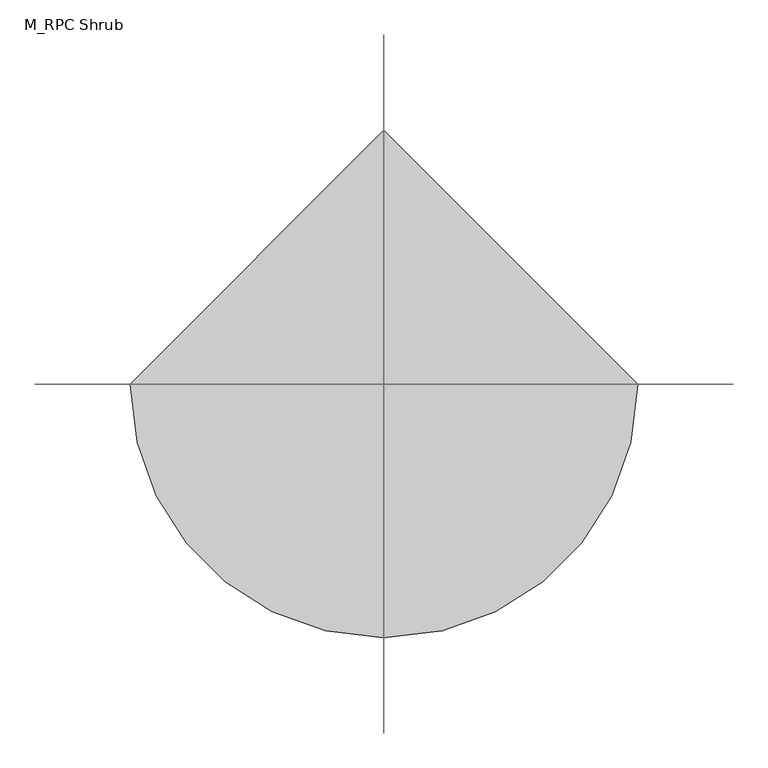
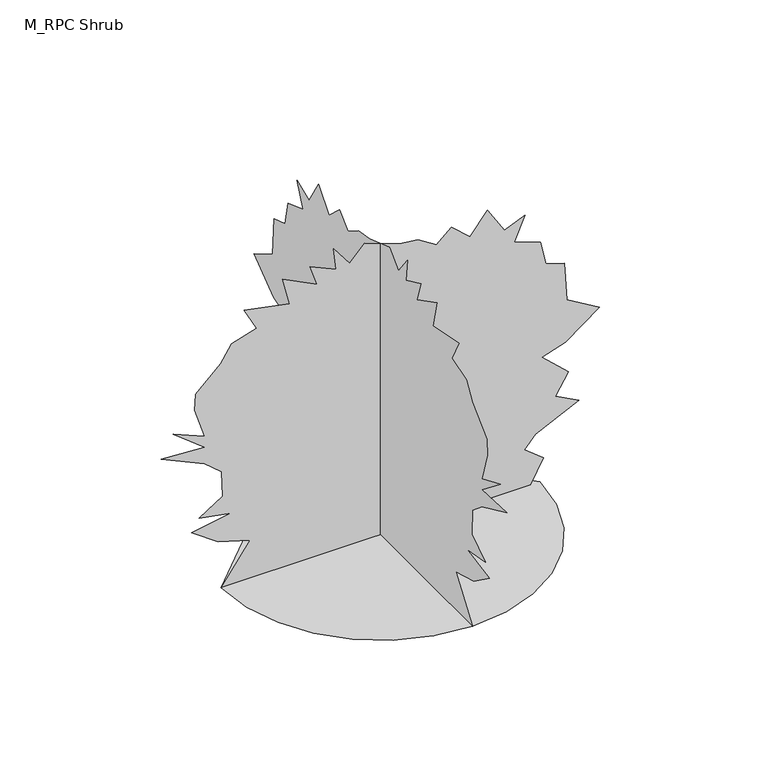
"""IFC4 building model written with IfcOpenShell, lengths in millimetres: geographic element geometry, M_RPC Shrub : Oleander - 1.62 Meters."""

import ifcopenshell
import ifcopenshell.guid

model = None  # the IFC model being written
_history = None  # IfcOwnerHistory: only IFC2X3 demands one
_inside = {}  # id of a spatial element -> (the spatial element, [elements in it])
_under = {}  # id of a project, library or spatial element -> (it, [spatial elements below it])
_declared = {}  # id of a project -> (the project, [libraries it declares])
_typed = {}  # id of a type object -> (the type object, [elements of that type])
_made_of = {}  # id of a material, layer set ... -> (it, [elements and type objects made of it])


def new_model(schema):
    """Start an empty IFC model of exactly this schema.

    Asked for "IFC4X3", IfcOpenShell would pick the latest addendum, in which some entities
    have other attributes; the version numbers below select the first issue.
    IFC2X3 requires an IfcOwnerHistory on every rooted entity: one is made here for all.
    """
    global model, _history
    if schema == "IFC4X3":
        model = ifcopenshell.file(schema_version=(4, 3, 0, 0))
    else:
        model = ifcopenshell.file(schema=schema)
    _inside.clear()
    _under.clear()
    _declared.clear()
    _typed.clear()
    _made_of.clear()
    _history = None
    if model.schema == "IFC2X3":
        org = make("IfcOrganization", Name="unknown")
        user = make(
            "IfcPersonAndOrganization",
            ThePerson=make("IfcPerson", FamilyName="unknown"),
            TheOrganization=org,
        )
        app = make(
            "IfcApplication",
            ApplicationDeveloper=org,
            Version="unknown",
            ApplicationFullName="unknown",
            ApplicationIdentifier="unknown",
        )
        _history = make(
            "IfcOwnerHistory",
            OwningUser=user,
            OwningApplication=app,
            ChangeAction="ADDED",
            CreationDate=0,
        )
    return model


def make(cls, **values):
    """One entity of the class cls with the attributes given. An attribute that is None is left unset."""
    return model.create_entity(
        cls, **{name: value for name, value in values.items() if value is not None}
    )


def rooted(cls, **values):
    """An entity with a GlobalId (a new one), such as an element, a storey or a relation."""
    return make(cls, GlobalId=ifcopenshell.guid.new(), OwnerHistory=_history, **values)


def si_unit(unit_type, name, prefix=None):
    """IfcSIUnit, for example si_unit("LENGTHUNIT", "METRE", prefix="MILLI")."""
    return make("IfcSIUnit", UnitType=unit_type, Prefix=prefix, Name=name)


def assignment(units):
    """IfcUnitAssignment: the units of a project."""
    return None if units is None else make("IfcUnitAssignment", Units=units)


def point(xyz):
    """IfcCartesianPoint."""
    return None if xyz is None else make("IfcCartesianPoint", Coordinates=xyz)


def direction(xyz):
    """IfcDirection."""
    return None if xyz is None else make("IfcDirection", DirectionRatios=xyz)


def frame(location, z_axis=None, x_axis=None):
    """IfcAxis2Placement3D, a coordinate frame: its origin and axes. An axis left out is left unset."""
    return make(
        "IfcAxis2Placement3D",
        Location=point(location),
        Axis=direction(z_axis),
        RefDirection=direction(x_axis),
    )


def origin():
    """The frame at (0, 0, 0) with its axes left unset."""
    return frame((0.0, 0.0, 0.0))


def place(relative_to, where):
    """IfcLocalPlacement: puts the frame where relative to a parent placement (None: the world)."""
    return make(
        "IfcLocalPlacement", PlacementRelTo=relative_to, RelativePlacement=where
    )


def context(
    kind, dimensions, precision=None, world=None, true_north=None, identifier=None
):
    """IfcGeometricRepresentationContext, for example the 3D "Model" context."""
    return make(
        "IfcGeometricRepresentationContext",
        ContextIdentifier=identifier,
        ContextType=kind,
        CoordinateSpaceDimension=dimensions,
        Precision=precision,
        WorldCoordinateSystem=world,
        TrueNorth=true_north,
    )


def project(units=None, contexts=None):
    """IfcProject with its units and contexts."""
    return rooted(
        "IfcProject",
        Name="project",
        RepresentationContexts=contexts,
        UnitsInContext=assignment(units),
    )


def spatial(cls, under=None, at=None, **own):
    """A site, building, storey or space (cls), placed at a placement, below another one or the project."""
    s = rooted(cls, ObjectPlacement=at, **own)
    if under is not None:
        _under.setdefault(under.id(), (under, []))[1].append(s)
    return s


def point_list(points):
    """IfcCartesianPointList2D or 3D."""
    cls = (
        "IfcCartesianPointList2D" if len(points[0]) == 2 else "IfcCartesianPointList3D"
    )
    return make(cls, CoordList=points)


def triangles(points, corners, closed=None, point_numbers=None):
    """IfcTriangulatedFaceSet: each triangle names its three corners, points numbered from 1."""
    return make(
        "IfcTriangulatedFaceSet",
        Coordinates=point_list(points),
        Closed=closed,
        CoordIndex=corners,
        PnIndex=point_numbers,
    )


def shape(context_of_items, identifier, shape_type, items):
    """IfcShapeRepresentation: the items that make up one representation, for example the "Body"."""
    return make(
        "IfcShapeRepresentation",
        ContextOfItems=context_of_items,
        RepresentationIdentifier=identifier,
        RepresentationType=shape_type,
        Items=items,
    )


def source(mapping_origin, context_of_items, identifier, shape_type, items):
    """IfcRepresentationMap: a shape defined once, which mapped items show again and again."""
    return make(
        "IfcRepresentationMap",
        MappingOrigin=mapping_origin,
        MappedRepresentation=shape(context_of_items, identifier, shape_type, items),
    )


def transform(
    local_origin,
    x_axis=None,
    y_axis=None,
    z_axis=None,
    scale=None,
    scale2=None,
    scale3=None,
    uniform=True,
):
    """IfcCartesianTransformationOperator3D, or its non-uniform kind. x_axis, y_axis, z_axis: its Axis1, 2, 3."""
    if uniform:
        return make(
            "IfcCartesianTransformationOperator3D",
            Axis1=direction(x_axis),
            Axis2=direction(y_axis),
            LocalOrigin=point(local_origin),
            Scale=scale,
            Axis3=direction(z_axis),
        )
    return make(
        "IfcCartesianTransformationOperator3DnonUniform",
        Axis1=direction(x_axis),
        Axis2=direction(y_axis),
        LocalOrigin=point(local_origin),
        Scale=scale,
        Axis3=direction(z_axis),
        Scale2=scale2,
        Scale3=scale3,
    )


def mapped(mapping_source, mapping_target):
    """IfcMappedItem: shows the shape of a source again, moved by a transform."""
    return make(
        "IfcMappedItem", MappingSource=mapping_source, MappingTarget=mapping_target
    )


def made_of(thing, what):
    """Note that an element or type object is made of a material, layer set ...; save() writes the relation."""
    if what is not None:
        _made_of.setdefault(what.id(), (what, []))[1].append(thing)
    return thing


def element(
    cls,
    number,
    at=None,
    inside=None,
    cuts=None,
    type_object=None,
    material=None,
    context=None,
    identifier="Body",
    shape_type=None,
    held_by="IfcProductDefinitionShape",
    body=None,
    shapes=None,
    **own,
):
    """One element of the class cls, such as IfcWall. Its Tag is "e" and its number.

    at: its placement. inside: the storey or other place that contains it. cuts: it is an
    opening in that element (IfcRelVoidsElement). A single representation is given by context,
    identifier, shape_type and body (its items); several are given by shapes. held_by: the class
    of the entity that holds the representations. save() writes the other relations.
    """
    e = rooted(cls, Tag="e%d" % number, ObjectPlacement=at, **own)
    if body is not None:
        shapes = [shape(context, identifier, shape_type, body)]
    if shapes is not None:
        e.Representation = make(held_by, Representations=shapes)
    if inside is not None:
        _inside.setdefault(inside.id(), (inside, []))[1].append(e)
    if cuts is not None:
        rooted(
            "IfcRelVoidsElement", RelatingBuildingElement=cuts, RelatedOpeningElement=e
        )
    if type_object is not None:
        _typed.setdefault(type_object.id(), (type_object, []))[1].append(e)
    return made_of(e, material)


def aggregate(whole, parts):
    """IfcRelAggregates: a whole, such as a stair, and the parts it consists of."""
    return rooted("IfcRelAggregates", RelatingObject=whole, RelatedObjects=parts)


def save(model, path):
    """Write the relations noted so far, then the file.

    IfcRelAggregates (storeys below a building ...), IfcRelContainedInSpatialStructure (elements
    in a storey), IfcRelDefinesByType, IfcRelAssociatesMaterial and IfcRelDeclares: one each for
    every whole, place, type object, material and project.
    """
    for whole, parts in _under.values():
        aggregate(whole, parts)
    for where, things in _inside.values():
        rooted(
            "IfcRelContainedInSpatialStructure",
            RelatedElements=things,
            RelatingStructure=where,
        )
    for kind, things in _typed.values():
        rooted("IfcRelDefinesByType", RelatedObjects=things, RelatingType=kind)
    for what, things in _made_of.values():
        rooted("IfcRelAssociatesMaterial", RelatedObjects=things, RelatingMaterial=what)
    for by, libraries in _declared.values():
        rooted("IfcRelDeclares", RelatingContext=by, RelatedDefinitions=libraries)
    model.write(path)


def m_rpc_shrub_9f7608c0(model_context):
    return source(origin(), model_context, "Body", "Tessellation", [
        triangles([(-809.7417807, 0.0, 3.61e-05), (-788.3350204, -185.5390928, 3.61e-05), (-727.3673029, -355.9266395, 3.61e-05), (-631.7240129, -506.2829052, 3.61e-05), (-506.2829052, -631.7240129, 3.61e-05), (-355.9266395, -727.3673029, 3.61e-05), (-185.5390928, -788.3350204, 3.61e-05), (3.54e-05, -809.7417807, 3.61e-05), (185.5390928, -788.3350204, 3.61e-05), (355.9266395, -727.3673029, 3.61e-05), (506.2829052, -631.7240129, 3.61e-05), (631.7240129, -506.2829052, 3.61e-05), (727.3673029, -355.9266395, 3.61e-05), (788.3350204, -185.5390928, 3.61e-05), (809.7417807, 7.08e-05, 3.61e-05), (-0.0001062, 809.7417807, 3.61e-05), (-0.00426, -808.5039928, 0.0001204), (-0.0042561, -663.4380655, 203.8035848), (-0.0042523, -825.0482592, 250.5848863), (-0.0042473, -961.1383535, 348.4012267), (-0.0042493, -761.2531706, 382.4237866), (-0.004246, -922.8633642, 412.1938082), (-0.0042455, -803.7832054, 488.7438595), (-0.0042415, -808.0357075, 620.5814518), (-0.0042381, -893.0933064, 692.8815445), (-0.0042317, -1114.2409996, 794.9491516), (-0.0042354, -893.0933064, 782.189102), (-0.0042292, -1054.7009565, 909.7742649), (-0.0042337, -893.0933064, 841.7292177), (-0.0042282, -944.1258745, 999.0843658), (-0.0042257, -939.8733725, 1084.1419647), (-0.0042241, -812.2882095, 1203.2220509), (-0.0042223, -757.0006685, 1292.5321518), (-0.004223, -629.4155783, 1330.8071411), (-0.0042185, -693.2081234, 1449.8873726), (-0.0042233, -463.5553897, 1403.104763), (-0.0042185, -497.5779133, 1547.7023323), (-0.0042238, -323.2127569, 1458.3922314), (-0.0042201, -357.2353168, 1564.7123405), (-0.0042238, -225.3964165, 1505.1723701), (-0.0042202, -238.1549219, 1619.9999542), (-0.0042246, -157.3508424, 1513.679845), (-0.0042233, -80.7997737, 1594.4824711), (-0.0042279, 97.8196469, 1530.6898533), (-0.0042297, 191.3817231, 1517.9323471), (-0.0042328, 284.9453434, 1458.3922314), (-0.0042319, 361.4954129, 1526.4373512), (-0.0042359, 455.0579796, 1441.3797523), (-0.0042339, 544.3680805, 1551.9548344), (-0.0042392, 629.4256794, 1415.86474), (-0.0042395, 735.7457886, 1458.3922314), (-0.0042424, 680.4581749, 1335.0596432), (-0.0042458, 812.2983833, 1288.277179), (-0.00425, 842.0658251, 1160.692016), (-0.0042523, 935.6284281, 1130.9219582), (-0.0042584, 948.3884777, 931.0393187), (-0.0042638, 1114.24863, 833.2242136), (-0.004265, 939.8834736, 705.6390507), (-0.0042644, 820.8033875, 667.3640614), (-0.0042702, 956.8934818, 539.7789348), (-0.0042724, 888.8484346, 433.4562821), (-0.004276, 1007.9285208, 369.663737), (-0.0042759, 786.7808275, 263.343646), (-0.004277, 731.4932865, 199.5508284), (-0.0042807, 829.3083189, 122.9995053), (-0.0042834, 763.7768538, 0.0205149), (-808.5141666, 0.0043303, 0.0), (-663.4481667, 0.0043182, 203.8035848), (-825.0558168, 0.0043154, 250.5848863), (-961.1459839, 0.0043096, 348.4012267), (-761.2632717, 0.0043075, 382.4237866), (-922.8709219, 0.0043058, 412.1938082), (-803.7908358, 0.0043012, 488.7438595), (-808.0433378, 0.0042934, 620.5814518), (-893.1009367, 0.004289, 692.8790737), (-1114.24863, 0.004283, 794.9491516), (-893.1009367, 0.0042837, 782.189102), (-1054.7085869, 0.0042761, 909.7742649), (-893.1009367, 0.0042802, 841.7292177), (-944.1359756, 0.0042708, 999.0843658), (-939.8809301, 0.0042657, 1084.1419647), (-812.2983833, 0.0042586, 1203.2220509), (-757.0107697, 0.0042533, 1292.5321518), (-629.4256794, 0.004251, 1330.8071411), (-693.2182245, 0.0042439, 1449.8873726), (-463.5629837, 0.0042467, 1403.104763), (-497.5855073, 0.0042381, 1547.7023323), (-323.2203509, 0.0042434, 1458.3922314), (-357.2429109, 0.0042371, 1564.7123405), (-225.4047735, 0.0042406, 1505.1723701), (-238.1635333, 0.0042338, 1619.9999542), (-157.3594538, 0.0042401, 1513.679845), (-80.8083851, 0.0042353, 1594.4824711), (97.8110446, 0.0042391, 1530.6898533), (191.3731298, 0.0042398, 1517.9323471), (284.935206, 0.0042434, 1458.3922314), (361.4878189, 0.0042393, 1526.4373512), (455.0503856, 0.0042444, 1441.3797523), (544.3604865, 0.0042378, 1551.9548344), (629.4155783, 0.0042459, 1415.8622692), (735.7381582, 0.0042434, 1458.3922314), (680.4506172, 0.0042508, 1335.0596432), (812.2882095, 0.0042535, 1288.277179), (842.0582674, 0.0042612, 1160.692016), (935.6208704, 0.0042629, 1130.9219582), (948.3783766, 0.0042748, 931.0393187), (1114.2409996, 0.0042807, 833.2242136), (939.8733725, 0.0042883, 705.6390507), (820.7932137, 0.0042905, 667.3640614), (956.8858515, 0.0042982, 539.7789348), (888.8408043, 0.0043045, 433.4562821), (1007.9184196, 0.0043083, 369.663737), (786.7707264, 0.0043146, 263.343646), (731.4856562, 0.0043184, 199.550574), (829.3007612, 0.004323, 122.9995053), (763.7692234, 0.0043303, 0.0204414)], [[15, 16, 1], [14, 15, 1], [14, 1, 2], [13, 14, 2], [13, 2, 3], [13, 3, 4], [12, 13, 4], [11, 12, 4], [11, 4, 5], [11, 5, 6], [11, 6, 7], [11, 7, 8], [11, 8, 9], [11, 9, 10], [27, 28, 29], [25, 26, 27], [40, 41, 42], [21, 22, 23], [50, 51, 52], [19, 20, 21], [38, 39, 40], [36, 37, 38], [34, 35, 36], [61, 62, 63], [66, 17, 18], [56, 57, 58], [48, 49, 50], [18, 19, 21], [46, 47, 48], [64, 65, 66], [59, 60, 61], [56, 58, 59], [54, 55, 56], [42, 43, 44], [52, 53, 54], [54, 56, 59], [24, 25, 27], [48, 50, 52], [59, 61, 63], [52, 54, 59], [48, 52, 59], [46, 48, 59], [66, 18, 21], [30, 31, 32], [29, 30, 32], [66, 21, 23], [66, 23, 24], [64, 66, 24], [63, 64, 24], [59, 63, 24], [46, 59, 24], [45, 46, 24], [44, 45, 24], [42, 44, 24], [40, 42, 24], [38, 40, 24], [36, 38, 24], [34, 36, 24], [34, 24, 27], [34, 27, 29], [34, 29, 32], [33, 34, 32], [77, 78, 79], [75, 76, 77], [90, 91, 92], [71, 72, 73], [100, 101, 102], [69, 70, 71], [88, 89, 90], [86, 87, 88], [84, 85, 86], [111, 112, 113], [116, 67, 68], [106, 107, 108], [98, 99, 100], [68, 69, 71], [96, 97, 98], [114, 115, 116], [109, 110, 111], [106, 108, 109], [104, 105, 106], [92, 93, 94], [102, 103, 104], [104, 106, 109], [74, 75, 77], [98, 100, 102], [109, 111, 113], [102, 104, 109], [98, 102, 109], [96, 98, 109], [116, 68, 71], [80, 81, 82], [79, 80, 82], [116, 71, 73], [116, 73, 74], [114, 116, 74], [113, 114, 74], [109, 113, 74], [96, 109, 74], [95, 96, 74], [94, 95, 74], [92, 94, 74], [90, 92, 74], [88, 90, 74], [86, 88, 74], [84, 86, 74], [84, 74, 77], [84, 77, 79], [84, 79, 82], [83, 84, 82]], closed=False),
    ])


if __name__ == "__main__":
    model = new_model("IFC4")
    model_context = context("Model", 3, world=origin())
    ifc_project = project(units=[si_unit("LENGTHUNIT", "METRE", prefix="MILLI")], contexts=[model_context])
    site = spatial("IfcSite", under=ifc_project)
    building = spatial("IfcBuilding", under=site)
    placement = place(None, origin())
    m_rpc_shrub_shape = m_rpc_shrub_9f7608c0(model_context)
    element("IfcGeographicElement", 1, ObjectType="M_RPC Shrub : Oleander - 1.62 Meters", at=placement, inside=building, context=model_context, shape_type="MappedRepresentation", body=[
        mapped(m_rpc_shrub_shape, transform((0.0, 0.0, 0.0), x_axis=(1.0, 0.0, 0.0), y_axis=(0.0, 1.0, 0.0), z_axis=(0.0, 0.0, 1.0))),
    ])
    save(model, "model.ifc")

# Revit data of these elements
# Type "M_RPC Shrub : Oleander - 1.62 Meters"
#   Type Comments = "Oleander"
#   built-in parameter 1005198 = "{2, 15},{39, RPC-16-G3GJ-A6PX-PK1P-U000-ST1L-LVER-AU},{1, 0},{1, 0},{2, 35},{1, 8},{5, Color},{1, 0},{1, 0},{3, 0.8},{3, 0.8},{3, 0.8},{1, 8},{7, BBoxMin},{1, 0},{1, 0},{1, 0},{1, 0},{1, 0},{1, 8},{7, BBoxMax},{1, 0},{1, 0},{1, 0},{1, 0},{1, 0},{2, 11},{9, RPCTypeId},{1, 0},{1, 0},{39, RPC-16-G3GJ-A6PX-PK1P-U000-ST1L-LVER-AU},{1, 6},{14, RPCPlantHeight},{1, 0},{1, 0},{7, 5.31496},{2, 11},{7, keyword},{1, 0},{1, 0},{22, :Geometry:RPC:Oleander},{2, 11},{8, category},{1, 0},{1, 0},{17, :Shrubs & Grasses},{2, 11},{12, LocalizedUID},{1, 0},{1, 0},{8, Oleander},{2, 14},{6, Height},{1, 0},{1, 0},{7, 5.31496},{1, 2},{16, Cast Reflections},{1, 0},{1, 0},{1, 0},{1, 2},{12, Cast Shadows},{1, 0},{1, 0},{1, 1},{1, 2},{9, Lock View},{1, 0},{1, 0},{1, 0},{1, 4},{5, ViewC},{1, 0},{1, 0},{1, 0},{2, 11},{20, AdvancedUIDefinition},{1, 0},{1, 0},{0, },{2, 11},{10, AssetLibID},{1, 0},{1, 0},{36, 4D3F6E72-3F99-4203-98E9-AF80B3C7A7A4},{2, 11},{10, BaseSchema},{1, 0},{1, 0},{9, RPCSchema},{2, 11},{12, ExchangeGUID},{1, 0},{1, 0},{0, },{1, 2},{6, Hidden},{1, 0},{1, 0},{1, 0},{1, 4},{11, RPCCategory},{1, 0},{1, 0},{1, 0},{2, 11},{8, RPCImage},{1, 0},{1, 0},{0, },{1, 4},{13, SchemaVersion},{1, 0},{1, 0},{1, 4},{2, 11},{12, UIDefinition},{1, 0},{1, 0},{0, },{2, 11},{6, UIName},{1, 0},{1, 0},{39, RPC-16-G3GJ-A6PX-PK1P-U000-ST1L-LVER-AU},{2, 11},{11, VersionGUID},{1, 0},{1, 0},{9, RPCSchema},{2, 11},{9, assettype},{1, 0},{1, 0},{11, RPCGeometry},{2, 11},{11, description},{1, 0},{1, 0},{0, },{2, 11},{9, localname},{1, 0},{1, 0},{3, RPC},{2, 11},{9, localtype},{1, 0},{1, 0},{3, RPC},{1, 4},{8, revision},{1, 0},{1, 0},{1, 1},{2, 11},{9, thumbnail},{1, 0},{1, 0},{0, },{1, 4},{7, version},{1, 0},{1, 0},{1, 1},{1, 2},{20, RPC_Cast Reflections},{1, 0},{1, 0},{1, 1},{1, 2},{16, RPC_Cast Shadows},{1, 0},{1, 0},{1, 1},{1, 2},{13, RPC_Lock View},{1, 0},{1, 0},{1, 0},{1, 4},{9, RPC_ViewC},{1, 0},{1, 0},{1, 0},{21, assetlibrary_base.fbx},{1, 5},"
#   built-in parameter 1005195 = "RPC-16-G3GJ-A6PX-PK1P-U000-ST1L-LVER-AU"
#   Height = 1.62 m
#   Description = (empty or 0)
